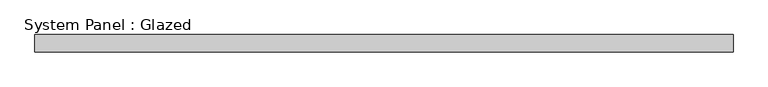
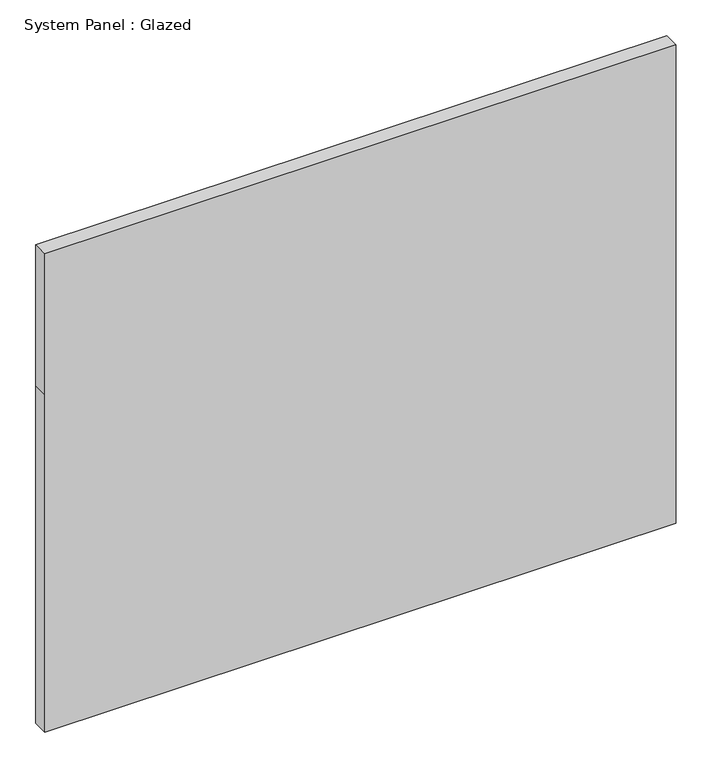
"""IFC4 building model written with IfcOpenShell, lengths in millimetres: plate geometry, System Panel : Glazed."""

from ifc_helpers import new_model, si_unit, frame, origin, place, context, project, spatial, polyline, outline, extrude, source, transform, mapped, element, save


def system_panel_glazed_13ee93ae(model_context):
    return source(origin(), model_context, "Body", "SweptSolid", [
        extrude(outline(polyline([(0.0, -511.4925), (0.0, 511.4925), (577.85, 511.4925), (819.15, 511.4925), (819.15, -511.4925), (577.85, -511.4925), (0.0, -511.4925)])), frame((0.0, -44.45, 0.0), z_axis=(0.0, 1.0, 0.0), x_axis=(0.0, 0.0, 1.0)), (0.0, 0.0, 1.0), 25.4),
    ])


if __name__ == "__main__":
    model = new_model("IFC4")
    model_context = context("Model", 3, world=origin())
    ifc_project = project(units=[si_unit("LENGTHUNIT", "METRE", prefix="MILLI")], contexts=[model_context])
    site = spatial("IfcSite", under=ifc_project)
    building = spatial("IfcBuilding", under=site)
    placement = place(None, origin())
    system_panel_glazed_shape = system_panel_glazed_13ee93ae(model_context)
    element("IfcPlate", 1, ObjectType="System Panel : Glazed", at=placement, inside=building, context=model_context, shape_type="MappedRepresentation", body=[
        mapped(system_panel_glazed_shape, transform((0.0, 0.0, 0.0), x_axis=(1.0, 0.0, 0.0), y_axis=(0.0, 1.0, 0.0), z_axis=(0.0, 0.0, 1.0))),
    ])
    save(model, "model.ifc")

# Revit data of these elements
# Element 1 (IfcPlate, "System Panel : Glazed")
#   Materials on its faces: "Glass"
# Materials
#   "Glass": class "Unassigned", colour RGB 147 173 200, transparency 0.7, Cost = 0
